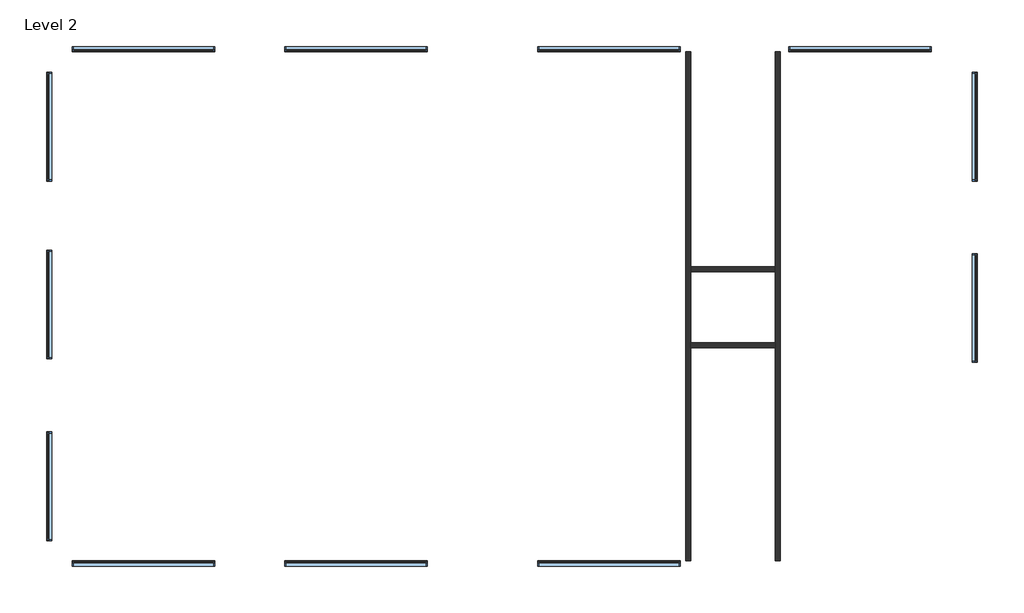
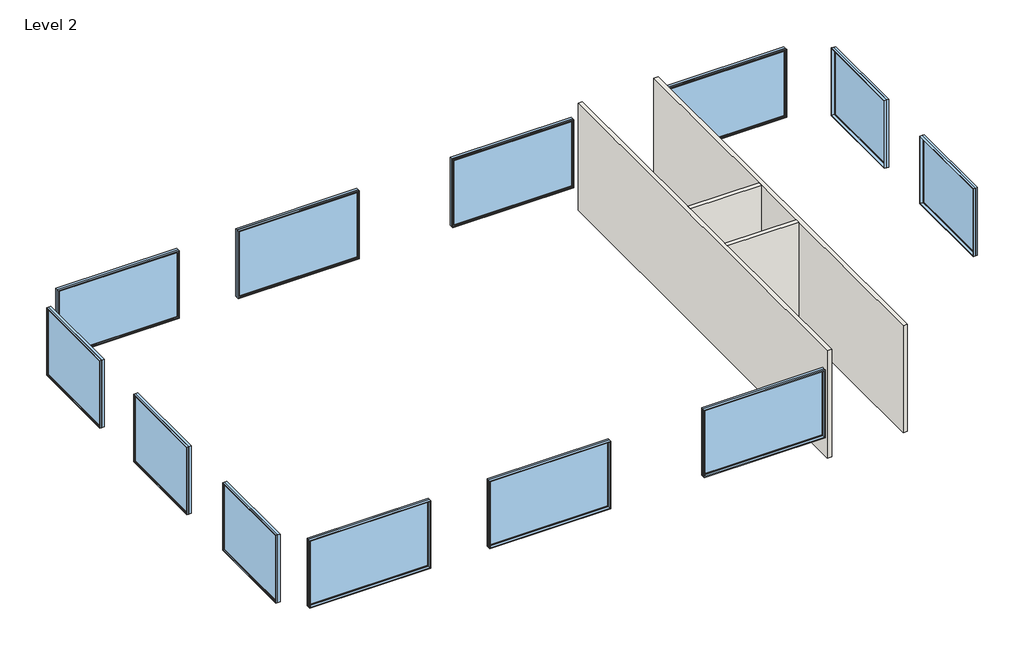
# One storey: 12 windows, 4 walls.
"""IFC4 building model written with IfcOpenShell, lengths in millimetres."""

import ifcopenshell
import ifcopenshell.guid

model = None  # the IFC model being written
_history = None  # IfcOwnerHistory: only IFC2X3 demands one
_inside = {}  # id of a spatial element -> (the spatial element, [elements in it])
_under = {}  # id of a project, library or spatial element -> (it, [spatial elements below it])
_declared = {}  # id of a project -> (the project, [libraries it declares])
_typed = {}  # id of a type object -> (the type object, [elements of that type])
_made_of = {}  # id of a material, layer set ... -> (it, [elements and type objects made of it])


def new_model(schema):
    """Start an empty IFC model of exactly this schema.

    Asked for "IFC4X3", IfcOpenShell would pick the latest addendum, in which some entities
    have other attributes; the version numbers below select the first issue.
    IFC2X3 requires an IfcOwnerHistory on every rooted entity: one is made here for all.
    """
    global model, _history
    if schema == "IFC4X3":
        model = ifcopenshell.file(schema_version=(4, 3, 0, 0))
    else:
        model = ifcopenshell.file(schema=schema)
    _inside.clear()
    _under.clear()
    _declared.clear()
    _typed.clear()
    _made_of.clear()
    _history = None
    if model.schema == "IFC2X3":
        org = make("IfcOrganization", Name="unknown")
        user = make(
            "IfcPersonAndOrganization",
            ThePerson=make("IfcPerson", FamilyName="unknown"),
            TheOrganization=org,
        )
        app = make(
            "IfcApplication",
            ApplicationDeveloper=org,
            Version="unknown",
            ApplicationFullName="unknown",
            ApplicationIdentifier="unknown",
        )
        _history = make(
            "IfcOwnerHistory",
            OwningUser=user,
            OwningApplication=app,
            ChangeAction="ADDED",
            CreationDate=0,
        )
    return model


def make(cls, **values):
    """One entity of the class cls with the attributes given. An attribute that is None is left unset."""
    return model.create_entity(
        cls, **{name: value for name, value in values.items() if value is not None}
    )


def rooted(cls, **values):
    """An entity with a GlobalId (a new one), such as an element, a storey or a relation."""
    return make(cls, GlobalId=ifcopenshell.guid.new(), OwnerHistory=_history, **values)


def si_unit(unit_type, name, prefix=None):
    """IfcSIUnit, for example si_unit("LENGTHUNIT", "METRE", prefix="MILLI")."""
    return make("IfcSIUnit", UnitType=unit_type, Prefix=prefix, Name=name)


def assignment(units):
    """IfcUnitAssignment: the units of a project."""
    return None if units is None else make("IfcUnitAssignment", Units=units)


def point(xyz):
    """IfcCartesianPoint."""
    return None if xyz is None else make("IfcCartesianPoint", Coordinates=xyz)


def direction(xyz):
    """IfcDirection."""
    return None if xyz is None else make("IfcDirection", DirectionRatios=xyz)


def frame(location, z_axis=None, x_axis=None):
    """IfcAxis2Placement3D, a coordinate frame: its origin and axes. An axis left out is left unset."""
    return make(
        "IfcAxis2Placement3D",
        Location=point(location),
        Axis=direction(z_axis),
        RefDirection=direction(x_axis),
    )


def origin():
    """The frame at (0, 0, 0) with its axes left unset."""
    return frame((0.0, 0.0, 0.0))


def place(relative_to, where):
    """IfcLocalPlacement: puts the frame where relative to a parent placement (None: the world)."""
    return make(
        "IfcLocalPlacement", PlacementRelTo=relative_to, RelativePlacement=where
    )


def context(
    kind, dimensions, precision=None, world=None, true_north=None, identifier=None
):
    """IfcGeometricRepresentationContext, for example the 3D "Model" context."""
    return make(
        "IfcGeometricRepresentationContext",
        ContextIdentifier=identifier,
        ContextType=kind,
        CoordinateSpaceDimension=dimensions,
        Precision=precision,
        WorldCoordinateSystem=world,
        TrueNorth=true_north,
    )


def project(units=None, contexts=None):
    """IfcProject with its units and contexts."""
    return rooted(
        "IfcProject",
        Name="project",
        RepresentationContexts=contexts,
        UnitsInContext=assignment(units),
    )


def spatial(cls, under=None, at=None, **own):
    """A site, building, storey or space (cls), placed at a placement, below another one or the project."""
    s = rooted(cls, ObjectPlacement=at, **own)
    if under is not None:
        _under.setdefault(under.id(), (under, []))[1].append(s)
    return s


def polyline(points):
    """IfcPolyline through the points."""
    return make("IfcPolyline", Points=[point(p) for p in points])


def outline(outer, holes=None, kind="AREA"):
    """IfcArbitraryClosedProfileDef: a profile drawn as a closed curve; with holes, ...WithVoids."""
    if holes is None:
        return make("IfcArbitraryClosedProfileDef", ProfileType=kind, OuterCurve=outer)
    return make(
        "IfcArbitraryProfileDefWithVoids",
        ProfileType=kind,
        OuterCurve=outer,
        InnerCurves=holes,
    )


def extrude(swept, where, along, depth):
    """IfcExtrudedAreaSolid: the profile swept, set in the frame where, extruded along a direction by depth."""
    return make(
        "IfcExtrudedAreaSolid",
        SweptArea=swept,
        Position=where,
        ExtrudedDirection=direction(along),
        Depth=depth,
    )


def faces_of(points, faces, orient=None, outer=None):
    """IfcFace entities. A face is a list of loops; a loop is a list of indices into points, from 0.

    orient and outer hold one flag for each loop. By default every Orientation is true, the
    first loop of a face is its IfcFaceOuterBound and the others are IfcFaceBound.
    """
    made = []
    for i, loops in enumerate(faces):
        bounds = []
        for j, loop in enumerate(loops):
            is_outer = j == 0 if outer is None else outer[i][j]
            bounds.append(
                make(
                    "IfcFaceOuterBound" if is_outer else "IfcFaceBound",
                    Bound=make("IfcPolyLoop", Polygon=[points[k] for k in loop]),
                    Orientation=True if orient is None else orient[i][j],
                )
            )
        made.append(make("IfcFace", Bounds=bounds))
    return made


def faceted_brep(points, faces, orient=None, outer=None, voids=None):
    """IfcFacetedBrep: a solid bounded by flat faces; with voids (closed shells), ...WithVoids."""
    shared = [point(p) for p in points]
    hull = make("IfcClosedShell", CfsFaces=faces_of(shared, faces, orient, outer))
    if voids is None:
        return make("IfcFacetedBrep", Outer=hull)
    return make(
        "IfcFacetedBrepWithVoids",
        Outer=hull,
        Voids=[
            make(cls, CfsFaces=faces_of(shared, fs, o, b)) for cls, fs, o, b in voids
        ],
    )


def shape(context_of_items, identifier, shape_type, items):
    """IfcShapeRepresentation: the items that make up one representation, for example the "Body"."""
    return make(
        "IfcShapeRepresentation",
        ContextOfItems=context_of_items,
        RepresentationIdentifier=identifier,
        RepresentationType=shape_type,
        Items=items,
    )


def source(mapping_origin, context_of_items, identifier, shape_type, items):
    """IfcRepresentationMap: a shape defined once, which mapped items show again and again."""
    return make(
        "IfcRepresentationMap",
        MappingOrigin=mapping_origin,
        MappedRepresentation=shape(context_of_items, identifier, shape_type, items),
    )


def transform(
    local_origin,
    x_axis=None,
    y_axis=None,
    z_axis=None,
    scale=None,
    scale2=None,
    scale3=None,
    uniform=True,
):
    """IfcCartesianTransformationOperator3D, or its non-uniform kind. x_axis, y_axis, z_axis: its Axis1, 2, 3."""
    if uniform:
        return make(
            "IfcCartesianTransformationOperator3D",
            Axis1=direction(x_axis),
            Axis2=direction(y_axis),
            LocalOrigin=point(local_origin),
            Scale=scale,
            Axis3=direction(z_axis),
        )
    return make(
        "IfcCartesianTransformationOperator3DnonUniform",
        Axis1=direction(x_axis),
        Axis2=direction(y_axis),
        LocalOrigin=point(local_origin),
        Scale=scale,
        Axis3=direction(z_axis),
        Scale2=scale2,
        Scale3=scale3,
    )


def mapped(mapping_source, mapping_target):
    """IfcMappedItem: shows the shape of a source again, moved by a transform."""
    return make(
        "IfcMappedItem", MappingSource=mapping_source, MappingTarget=mapping_target
    )


def made_of(thing, what):
    """Note that an element or type object is made of a material, layer set ...; save() writes the relation."""
    if what is not None:
        _made_of.setdefault(what.id(), (what, []))[1].append(thing)
    return thing


def element(
    cls,
    number,
    at=None,
    inside=None,
    cuts=None,
    type_object=None,
    material=None,
    context=None,
    identifier="Body",
    shape_type=None,
    held_by="IfcProductDefinitionShape",
    body=None,
    shapes=None,
    **own,
):
    """One element of the class cls, such as IfcWall. Its Tag is "e" and its number.

    at: its placement. inside: the storey or other place that contains it. cuts: it is an
    opening in that element (IfcRelVoidsElement). A single representation is given by context,
    identifier, shape_type and body (its items); several are given by shapes. held_by: the class
    of the entity that holds the representations. save() writes the other relations.
    """
    e = rooted(cls, Tag="e%d" % number, ObjectPlacement=at, **own)
    if body is not None:
        shapes = [shape(context, identifier, shape_type, body)]
    if shapes is not None:
        e.Representation = make(held_by, Representations=shapes)
    if inside is not None:
        _inside.setdefault(inside.id(), (inside, []))[1].append(e)
    if cuts is not None:
        rooted(
            "IfcRelVoidsElement", RelatingBuildingElement=cuts, RelatedOpeningElement=e
        )
    if type_object is not None:
        _typed.setdefault(type_object.id(), (type_object, []))[1].append(e)
    return made_of(e, material)


def aggregate(whole, parts):
    """IfcRelAggregates: a whole, such as a stair, and the parts it consists of."""
    return rooted("IfcRelAggregates", RelatingObject=whole, RelatedObjects=parts)


def save(model, path):
    """Write the relations noted so far, then the file.

    IfcRelAggregates (storeys below a building ...), IfcRelContainedInSpatialStructure (elements
    in a storey), IfcRelDefinesByType, IfcRelAssociatesMaterial and IfcRelDeclares: one each for
    every whole, place, type object, material and project.
    """
    for whole, parts in _under.values():
        aggregate(whole, parts)
    for where, things in _inside.values():
        rooted(
            "IfcRelContainedInSpatialStructure",
            RelatedElements=things,
            RelatingStructure=where,
        )
    for kind, things in _typed.values():
        rooted("IfcRelDefinesByType", RelatedObjects=things, RelatingType=kind)
    for what, things in _made_of.values():
        rooted("IfcRelAssociatesMaterial", RelatedObjects=things, RelatingMaterial=what)
    for by, libraries in _declared.values():
        rooted("IfcRelDeclares", RelatingContext=by, RelatedDefinitions=libraries)
    model.write(path)


def m_fixed_2500x_4228mm_fd5e51e7(model_context):
    return source(origin(), model_context, "Body", "SweptSolid", [
        extrude(outline(polyline([(-2050.8, 54.2), (2050.8, 54.2), (2050.8, 42.2), (-2050.8, 42.2), (-2050.8, 54.2)])), frame((0.0, 0.0, 368.0), z_axis=(0.0, 0.0, 1.0), x_axis=(1.0, 0.0, 0.0)), (0.0, 0.0, 1.0), 2374.0),
        extrude(outline(polyline([(2786.0, -2094.8), (324.0, -2094.8), (324.0, 2094.8), (2786.0, 2094.8), (2786.0, -2094.8)]), holes=[polyline([(2742.0, -2050.8), (2742.0, 2050.8), (368.0, 2050.8), (368.0, -2050.8), (2742.0, -2050.8)])]), frame((0.0, 26.2, 0.0), z_axis=(0.0, 1.0, 0.0), x_axis=(0.0, 0.0, 1.0)), (0.0, 0.0, 1.0), 44.0),
        extrude(outline(polyline([(2805.0, -2113.8), (305.0, -2113.8), (305.0, 2113.8), (2805.0, 2113.8), (2805.0, -2113.8)]), holes=[polyline([(2786.0, -2094.8), (2786.0, 2094.8), (324.0, 2094.8), (324.0, -2094.8), (2786.0, -2094.8)])]), frame((0.0, 26.2, 0.0), z_axis=(0.0, 1.0, 0.0), x_axis=(0.0, 0.0, 1.0)), (0.0, 0.0, 1.0), 63.0),
        extrude(outline(polyline([(2805.0, -2113.8), (305.0, -2113.8), (305.0, 2113.8), (2805.0, 2113.8), (2805.0, -2113.8)]), holes=[polyline([(2773.0, -2081.8), (2773.0, 2081.8), (337.0, 2081.8), (337.0, -2081.8), (2773.0, -2081.8)])]), frame((0.0, -63.2, 0.0), z_axis=(0.0, 1.0, 0.0), x_axis=(0.0, 0.0, 1.0)), (0.0, 0.0, 1.0), 89.4),
    ])


def m_fixed_2500x_4228mm_f14c179f(model_context):
    return source(origin(), model_context, "Body", "SweptSolid", [
        extrude(outline(polyline([(-2050.8, -54.2), (-2050.8, -42.2), (2050.8, -42.2), (2050.8, -54.2), (-2050.8, -54.2)])), frame((0.0, 0.0, 368.0), z_axis=(0.0, 0.0, 1.0), x_axis=(1.0, 0.0, 0.0)), (0.0, 0.0, 1.0), 2374.0),
        extrude(outline(polyline([(2786.0, -2094.8), (324.0, -2094.8), (324.0, 2094.8), (2786.0, 2094.8), (2786.0, -2094.8)]), holes=[polyline([(2742.0, -2050.8), (2742.0, 2050.8), (368.0, 2050.8), (368.0, -2050.8), (2742.0, -2050.8)])]), frame((0.0, -70.2, 0.0), z_axis=(0.0, 1.0, 0.0), x_axis=(0.0, 0.0, 1.0)), (0.0, 0.0, 1.0), 44.0),
        extrude(outline(polyline([(2805.0, -2113.8), (305.0, -2113.8), (305.0, 2113.8), (2805.0, 2113.8), (2805.0, -2113.8)]), holes=[polyline([(2786.0, -2094.8), (2786.0, 2094.8), (324.0, 2094.8), (324.0, -2094.8), (2786.0, -2094.8)])]), frame((0.0, -89.2, 0.0), z_axis=(0.0, 1.0, 0.0), x_axis=(0.0, 0.0, 1.0)), (0.0, 0.0, 1.0), 63.0),
        extrude(outline(polyline([(2805.0, -2113.8), (305.0, -2113.8), (305.0, 2113.8), (2805.0, 2113.8), (2805.0, -2113.8)]), holes=[polyline([(2773.0, -2081.8), (2773.0, 2081.8), (337.0, 2081.8), (337.0, -2081.8), (2773.0, -2081.8)])]), frame((0.0, -26.2, 0.0), z_axis=(0.0, 1.0, 0.0), x_axis=(0.0, 0.0, 1.0)), (0.0, 0.0, 1.0), 89.4),
    ])


def m_fixed_2500x_3220mm_df94f4d0(model_context):
    return source(origin(), model_context, "Body", "SweptSolid", [
        extrude(outline(polyline([(-1546.8, 54.2), (1546.8, 54.2), (1546.8, 42.2), (-1546.8, 42.2), (-1546.8, 54.2)])), frame((0.0, 0.0, 368.0), z_axis=(0.0, 0.0, 1.0), x_axis=(1.0, 0.0, 0.0)), (0.0, 0.0, 1.0), 2374.0),
        extrude(outline(polyline([(2786.0, -1590.8), (324.0, -1590.8), (324.0, 1590.8), (2786.0, 1590.8), (2786.0, -1590.8)]), holes=[polyline([(2742.0, -1546.8), (2742.0, 1546.8), (368.0, 1546.8), (368.0, -1546.8), (2742.0, -1546.8)])]), frame((0.0, 26.2, 0.0), z_axis=(0.0, 1.0, 0.0), x_axis=(0.0, 0.0, 1.0)), (0.0, 0.0, 1.0), 44.0),
        extrude(outline(polyline([(2805.0, -1609.8), (305.0, -1609.8), (305.0, 1609.8), (2805.0, 1609.8), (2805.0, -1609.8)]), holes=[polyline([(2786.0, -1590.8), (2786.0, 1590.8), (324.0, 1590.8), (324.0, -1590.8), (2786.0, -1590.8)])]), frame((0.0, 26.2, 0.0), z_axis=(0.0, 1.0, 0.0), x_axis=(0.0, 0.0, 1.0)), (0.0, 0.0, 1.0), 63.0),
        extrude(outline(polyline([(2805.0, -1609.8), (305.0, -1609.8), (305.0, 1609.8), (2805.0, 1609.8), (2805.0, -1609.8)]), holes=[polyline([(2773.0, -1577.8), (2773.0, 1577.8), (337.0, 1577.8), (337.0, -1577.8), (2773.0, -1577.8)])]), frame((0.0, -63.2, 0.0), z_axis=(0.0, 1.0, 0.0), x_axis=(0.0, 0.0, 1.0)), (0.0, 0.0, 1.0), 89.4),
    ])


def m_fixed_2500x_3220mm_8b997f8c(model_context):
    return source(origin(), model_context, "Body", "SweptSolid", [
        extrude(outline(polyline([(-1546.8, -54.2), (-1546.8, -42.2), (1546.8, -42.2), (1546.8, -54.2), (-1546.8, -54.2)])), frame((0.0, 0.0, 368.0), z_axis=(0.0, 0.0, 1.0), x_axis=(1.0, 0.0, 0.0)), (0.0, 0.0, 1.0), 2374.0),
        extrude(outline(polyline([(2786.0, -1590.8), (324.0, -1590.8), (324.0, 1590.8), (2786.0, 1590.8), (2786.0, -1590.8)]), holes=[polyline([(2742.0, -1546.8), (2742.0, 1546.8), (368.0, 1546.8), (368.0, -1546.8), (2742.0, -1546.8)])]), frame((0.0, -70.2, 0.0), z_axis=(0.0, 1.0, 0.0), x_axis=(0.0, 0.0, 1.0)), (0.0, 0.0, 1.0), 44.0),
        extrude(outline(polyline([(2805.0, -1609.8), (305.0, -1609.8), (305.0, 1609.8), (2805.0, 1609.8), (2805.0, -1609.8)]), holes=[polyline([(2786.0, -1590.8), (2786.0, 1590.8), (324.0, 1590.8), (324.0, -1590.8), (2786.0, -1590.8)])]), frame((0.0, -89.2, 0.0), z_axis=(0.0, 1.0, 0.0), x_axis=(0.0, 0.0, 1.0)), (0.0, 0.0, 1.0), 63.0),
        extrude(outline(polyline([(2805.0, -1609.8), (305.0, -1609.8), (305.0, 1609.8), (2805.0, 1609.8), (2805.0, -1609.8)]), holes=[polyline([(2773.0, -1577.8), (2773.0, 1577.8), (337.0, 1577.8), (337.0, -1577.8), (2773.0, -1577.8)])]), frame((0.0, -26.2, 0.0), z_axis=(0.0, 1.0, 0.0), x_axis=(0.0, 0.0, 1.0)), (0.0, 0.0, 1.0), 89.4),
    ])


model = new_model("IFC4")

# Units and contexts
model_context = context("Model", 3, world=origin())
ifc_project = project(units=[si_unit("LENGTHUNIT", "METRE", prefix="MILLI")], contexts=[model_context])

# Site, building, storey
site = spatial("IfcSite", under=ifc_project)
building = spatial("IfcBuilding", under=site)
storey = spatial("IfcBuildingStorey", under=building, Name="Level 2", Elevation=3962.4)

# Walls
placement = place(None, origin())
element("IfcWall", 1, ObjectType="Generic - 152.4mm - Interior", at=placement, inside=storey, context=model_context, shape_type="Brep", body=[
    faceted_brep([(20570.5967133, -3943.0197783, 3962.4), (20570.5967133, 2367.7802217, 3962.4), (20570.5967133, 2520.1802217, 3962.4), (20570.5967133, 4620.1802217, 3962.4), (20570.5967133, 4772.5802217, 3962.4), (20570.5967133, 11144.5802217, 3962.4), (20570.5967133, 11144.5802217, 7924.8), (20570.5967133, 4772.5802217, 7924.8), (20570.5967133, 4620.1802217, 7924.8), (20570.5967133, 2520.1802217, 7924.8), (20570.5967133, 2367.7802217, 7924.8), (20570.5967133, -3943.0197783, 7924.8), (20418.1967133, -3943.0197783, 3962.4), (20418.1967133, -3943.0197783, 7924.8), (20418.1967133, 11144.5802217, 7924.8), (20418.1967133, 11144.5802217, 3962.4)], [[[0, 1, 2, 3, 4, 5, 6, 7, 8, 9, 10, 11]], [[12, 13, 14, 15]], [[5, 4, 3, 2, 1, 0, 12, 15]], [[11, 10, 9, 8, 7, 6, 14, 13]], [[6, 5, 15, 14]], [[0, 11, 13, 12]]]),
])
element("IfcWall", 2, ObjectType="Generic - 152.4mm - Interior", at=placement, inside=storey, context=model_context, shape_type="Brep", body=[
    faceted_brep([(23222.9967133, -3943.0197783, 3962.4), (23222.9967133, 11144.5802217, 3962.4), (23222.9967133, 11144.5802217, 7924.8), (23222.9967133, -3943.0197783, 7924.8), (23070.5967133, -3943.0197783, 3962.4), (23070.5967133, -3943.0197783, 7924.8), (23070.5967133, 2367.7802217, 7924.8), (23070.5967133, 2520.1802217, 7924.8), (23070.5967133, 4620.1802217, 7924.8), (23070.5967133, 4772.5802217, 7924.8), (23070.5967133, 11144.5802217, 7924.8), (23070.5967133, 11144.5802217, 3962.4), (23070.5967133, 4772.5802217, 3962.4), (23070.5967133, 4620.1802217, 3962.4), (23070.5967133, 2520.1802217, 3962.4), (23070.5967133, 2367.7802217, 3962.4)], [[[0, 1, 2, 3]], [[4, 5, 6, 7, 8, 9, 10, 11, 12, 13, 14, 15]], [[1, 0, 4, 15, 14, 13, 12, 11]], [[3, 2, 10, 9, 8, 7, 6, 5]], [[2, 1, 11, 10]], [[0, 3, 5, 4]]]),
])
element("IfcWall", 3, ObjectType="Generic - 152.4mm - Interior", at=placement, inside=storey, context=model_context, shape_type="SweptSolid", body=[
    extrude(outline(polyline([(23070.5967133, 4620.1802217), (20570.5967133, 4620.1802217), (20570.5967133, 4772.5802217), (23070.5967133, 4772.5802217), (23070.5967133, 4620.1802217)])), frame((0.0, 0.0, 3962.4), z_axis=(0.0, 0.0, 1.0), x_axis=(1.0, 0.0, 0.0)), (0.0, 0.0, 1.0), 3962.4),
])
element("IfcWall", 4, ObjectType="Generic - 152.4mm - Interior", at=placement, inside=storey, context=model_context, shape_type="SweptSolid", body=[
    extrude(outline(polyline([(23070.5967133, 2367.7802217), (20570.5967133, 2367.7802217), (20570.5967133, 2520.1802217), (23070.5967133, 2520.1802217), (23070.5967133, 2367.7802217)])), frame((0.0, 0.0, 3962.4), z_axis=(0.0, 0.0, 1.0), x_axis=(1.0, 0.0, 0.0)), (0.0, 0.0, 1.0), 3962.4),
])

# Windows
m_fixed_2500x_4228mm_shape = m_fixed_2500x_4228mm_fd5e51e7(model_context)
element("IfcWindow", 5, ObjectType="M_Fixed : 2500X 4228mm", at=placement, inside=storey, context=model_context, shape_type="MappedRepresentation", body=[
    mapped(m_fixed_2500x_4228mm_shape, transform((4360.264681, 11233.7802217, 4557.4), x_axis=(-1.0, 0.0, 0.0), y_axis=(0.0, -1.0, 0.0), z_axis=(0.0, 0.0, 1.0))),
])
element("IfcWindow", 6, ObjectType="M_Fixed : 2500X 4228mm", at=placement, inside=storey, context=model_context, shape_type="MappedRepresentation", body=[
    mapped(m_fixed_2500x_4228mm_shape, transform((10652.264681, 11233.7802217, 4557.4), x_axis=(-1.0, 0.0, 0.0), y_axis=(0.0, -1.0, 0.0), z_axis=(0.0, 0.0, 1.0))),
])
element("IfcWindow", 7, ObjectType="M_Fixed : 2500X 4228mm", at=placement, inside=storey, context=model_context, shape_type="MappedRepresentation", body=[
    mapped(m_fixed_2500x_4228mm_shape, transform((18152.264681, 11233.7802217, 4557.4), x_axis=(-1.0, 0.0, 0.0), y_axis=(0.0, -1.0, 0.0), z_axis=(0.0, 0.0, 1.0))),
])
element("IfcWindow", 8, ObjectType="M_Fixed : 2500X 4228mm", at=placement, inside=storey, context=model_context, shape_type="MappedRepresentation", body=[
    mapped(m_fixed_2500x_4228mm_shape, transform((25592.264681, 11233.7802217, 4557.4), x_axis=(-1.0, 0.0, 0.0), y_axis=(0.0, -1.0, 0.0), z_axis=(0.0, 0.0, 1.0))),
])
m_fixed_2500x_4228mm_2_shape = m_fixed_2500x_4228mm_f14c179f(model_context)
element("IfcWindow", 9, ObjectType="M_Fixed : 2500X 4228mm", at=placement, inside=storey, context=model_context, shape_type="MappedRepresentation", body=[
    mapped(m_fixed_2500x_4228mm_2_shape, transform((4360.264681, -4032.2197783, 4557.4), x_axis=(-1.0, 0.0, 0.0), y_axis=(0.0, -1.0, 0.0), z_axis=(0.0, 0.0, 1.0))),
])
element("IfcWindow", 10, ObjectType="M_Fixed : 2500X 4228mm", at=placement, inside=storey, context=model_context, shape_type="MappedRepresentation", body=[
    mapped(m_fixed_2500x_4228mm_2_shape, transform((10652.264681, -4032.2197783, 4557.4), x_axis=(-1.0, 0.0, 0.0), y_axis=(0.0, -1.0, 0.0), z_axis=(0.0, 0.0, 1.0))),
])
element("IfcWindow", 11, ObjectType="M_Fixed : 2500X 4228mm", at=placement, inside=storey, context=model_context, shape_type="MappedRepresentation", body=[
    mapped(m_fixed_2500x_4228mm_2_shape, transform((18152.264681, -4032.2197783, 4557.4), x_axis=(-1.0, 0.0, 0.0), y_axis=(0.0, -1.0, 0.0), z_axis=(0.0, 0.0, 1.0))),
])
m_fixed_2500x_3220mm_shape = m_fixed_2500x_3220mm_df94f4d0(model_context)
element("IfcWindow", 12, ObjectType="M_Fixed : 2500x 3220mm", at=placement, inside=storey, context=model_context, shape_type="MappedRepresentation", body=[
    mapped(m_fixed_2500x_3220mm_shape, transform((1573.264681, 8920.7802217, 4559.8), x_axis=(0.0, 1.0, 0.0), y_axis=(-1.0, 0.0, 0.0), z_axis=(0.0, 0.0, 1.0))),
])
element("IfcWindow", 13, ObjectType="M_Fixed : 2500x 3220mm", at=placement, inside=storey, context=model_context, shape_type="MappedRepresentation", body=[
    mapped(m_fixed_2500x_3220mm_shape, transform((1573.264681, 3652.7802217, 4559.8), x_axis=(0.0, 1.0, 0.0), y_axis=(-1.0, 0.0, 0.0), z_axis=(0.0, 0.0, 1.0))),
])
element("IfcWindow", 14, ObjectType="M_Fixed : 2500x 3220mm", at=placement, inside=storey, context=model_context, shape_type="MappedRepresentation", body=[
    mapped(m_fixed_2500x_3220mm_shape, transform((1573.264681, -1733.2197783, 4559.8), x_axis=(0.0, 1.0, 0.0), y_axis=(-1.0, 0.0, 0.0), z_axis=(0.0, 0.0, 1.0))),
])
m_fixed_2500x_3220mm_2_shape = m_fixed_2500x_3220mm_8b997f8c(model_context)
element("IfcWindow", 15, ObjectType="M_Fixed : 2500x 3220mm", at=placement, inside=storey, context=model_context, shape_type="MappedRepresentation", body=[
    mapped(m_fixed_2500x_3220mm_2_shape, transform((28979.264681, 8920.7802217, 4559.8), x_axis=(0.0, 1.0, 0.0), y_axis=(-1.0, 0.0, 0.0), z_axis=(0.0, 0.0, 1.0))),
])
element("IfcWindow", 16, ObjectType="M_Fixed : 2500x 3220mm", at=placement, inside=storey, context=model_context, shape_type="MappedRepresentation", body=[
    mapped(m_fixed_2500x_3220mm_2_shape, transform((28979.264681, 3552.7802217, 4559.8), x_axis=(0.0, 1.0, 0.0), y_axis=(-1.0, 0.0, 0.0), z_axis=(0.0, 0.0, 1.0))),
])

save(model, "model.ifc")

# Revit data of these elements
# Type "Generic - 152.4mm - Interior"
#   Layers, outside or top first: 152.4 mm no material (function 1)
# Type "M_Fixed : 2500X 4228mm"
#   Type Mark = "25"
#   Height = 2500 mm
#   Default Sill Height = 305 mm
#   Width = 4227.6 mm
#   Window Inset = 19 mm
#   Frame Exterior Material = Sash
#   Frame Interior Material = Sash
#   Glass Pane Material = Glass
#   Sash = Sash
#   Wall Closure = (empty or 0)
# Type "M_Fixed : 2500x 3220mm"
#   Type Mark = "26"
#   Height = 2500 mm
#   Default Sill Height = 305 mm
#   Width = 3219.6 mm
#   Window Inset = 19 mm
#   Frame Exterior Material = Sash
#   Frame Interior Material = Sash
#   Glass Pane Material = Glass
#   Sash = Sash
#   Wall Closure = (empty or 0)
# Elements 1, 2, 3, 4 (IfcWall, "Generic - 152.4mm - Interior")
#   Top Offset = 0 mm
#   Base Offset = 0 mm
#   wall height = 3962.4 mm
#   Phase Created = New Construction
#   Base Constraint = Level 2
#   Top Constraint = Roof Level
#   Materials on its faces: "Default Wall"
# Element 5 (IfcWindow, "M_Fixed : 2500X 4228mm")
#   Mark = "1"
#   Phase Created = New Construction
#   Materials on its faces: "Sash", "Glass"
# Element 6 (IfcWindow, "M_Fixed : 2500X 4228mm")
#   Mark = "2"
#   Phase Created = New Construction
#   Materials on its faces: "Sash", "Glass"
# Element 7 (IfcWindow, "M_Fixed : 2500X 4228mm")
#   Mark = "3"
#   Phase Created = New Construction
#   Materials on its faces: "Sash", "Glass"
# Element 8 (IfcWindow, "M_Fixed : 2500X 4228mm")
#   Mark = "4"
#   Phase Created = New Construction
#   Materials on its faces: "Sash", "Glass"
# Element 9 (IfcWindow, "M_Fixed : 2500X 4228mm")
#   Mark = "5"
#   Phase Created = New Construction
#   Materials on its faces: "Sash", "Glass"
# Element 10 (IfcWindow, "M_Fixed : 2500X 4228mm")
#   Mark = "6"
#   Phase Created = New Construction
#   Materials on its faces: "Sash", "Glass"
# Element 11 (IfcWindow, "M_Fixed : 2500X 4228mm")
#   Mark = "7"
#   Phase Created = New Construction
#   Materials on its faces: "Sash", "Glass"
# Element 12 (IfcWindow, "M_Fixed : 2500x 3220mm")
#   Mark = "9"
#   Phase Created = New Construction
#   Materials on its faces: "Sash", "Glass"
# Element 13 (IfcWindow, "M_Fixed : 2500x 3220mm")
#   Mark = "18"
#   Phase Created = New Construction
#   Materials on its faces: "Sash", "Glass"
# Element 14 (IfcWindow, "M_Fixed : 2500x 3220mm")
#   Mark = "19"
#   Phase Created = New Construction
#   Materials on its faces: "Sash", "Glass"
# Element 15 (IfcWindow, "M_Fixed : 2500x 3220mm")
#   Mark = "20"
#   Phase Created = New Construction
#   Materials on its faces: "Sash", "Glass"
# Element 16 (IfcWindow, "M_Fixed : 2500x 3220mm")
#   Mark = "21"
#   Phase Created = New Construction
#   Materials on its faces: "Sash", "Glass"
# Materials
#   "Sash": class "Wood", colour RGB 136 99 55, transparency 0
#   "Glass": class "Glass", colour RGB 0 128 192, transparency 0.9, Description = "Soda Lime Glass", Cost = 0
#   "Default Wall": class "Miscellaneous", colour RGB 128 128 128, transparency 0, Cost = 0
# Room at (7702.307, 8283.876) mm, phase "New Construction", upper level "Roof Level", upper offset 0 mm, lower offset 0 mm
#   Number = "9"
#   Name = "Room"
# Room at (8641.307, 981.272) mm, phase "New Construction", upper level "Roof Level", upper offset 0 mm, lower offset 0 mm
#   Number = "10"
#   Name = "Room"
# Room at (17435.814, 4095.438) mm, phase "New Construction", upper level "Level 2", upper offset 3962.4 mm, lower offset 0 mm
#   Number = "11"
#   Name = "Room"
# Room at (21635.538, 7886.855) mm, phase "New Construction", upper level "Level 2", upper offset 3962.4 mm, lower offset 0 mm
#   Number = "12"
#   Name = "Room"
# Room at (26768.533, 4562.074) mm, phase "New Construction", upper level "Level 2", upper offset 3962.4 mm, lower offset 0 mm
#   Number = "13"
#   Name = "Room"
# Room at (21635.538, 0) mm, phase "New Construction", upper level "Level 2", upper offset 3962.4 mm, lower offset 0 mm
#   Number = "14"
#   Name = "Room"
